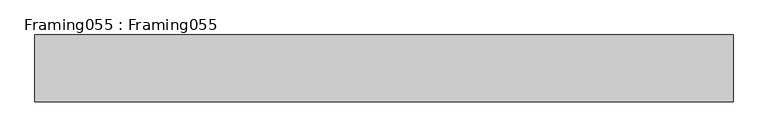
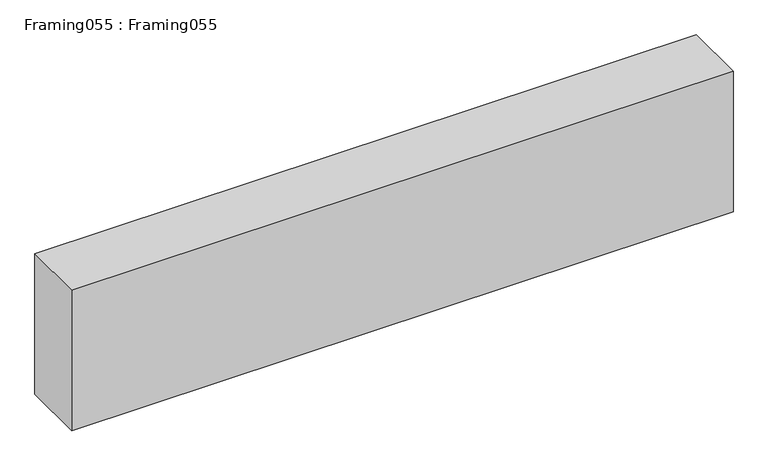
"""IFC4 building model written with IfcOpenShell, lengths in millimetres: proxy geometry, Framing055 : Framing055."""

from ifc_helpers import new_model, si_unit, frame, origin, place, context, project, spatial, polyline, outline, extrude, source, transform, mapped, element, save


def framing055_framing055_ac69ba7b(model_context):
    return source(origin(), model_context, "Body", "SweptSolid", [
        extrude(outline(polyline([(-5503.7121051, 9829.7531721), (-7089.7776325, 9829.7531721), (-7089.7776325, 9982.1531721), (-5503.7121051, 9982.1531721), (-5503.7121051, 9829.7531721)])), frame((0.0, 0.0, 39579.2960083), z_axis=(0.0, 0.0, 1.0), x_axis=(1.0, 0.0, 0.0)), (0.0, 0.0, 1.0), 355.6),
    ])


if __name__ == "__main__":
    model = new_model("IFC4")
    model_context = context("Model", 3, world=origin())
    ifc_project = project(units=[si_unit("LENGTHUNIT", "METRE", prefix="MILLI")], contexts=[model_context])
    site = spatial("IfcSite", under=ifc_project)
    building = spatial("IfcBuilding", under=site)
    placement = place(None, origin())
    framing055_framing055_shape = framing055_framing055_ac69ba7b(model_context)
    element("IfcBuildingElementProxy", 1, Name="Framing055 : Framing055", ObjectType="Framing055 : Framing055", at=placement, inside=building, context=model_context, shape_type="MappedRepresentation", body=[
        mapped(framing055_framing055_shape, transform((0.0, 0.0, 0.0), x_axis=(1.0, 0.0, 0.0), y_axis=(0.0, 1.0, 0.0), z_axis=(0.0, 0.0, 1.0))),
    ])
    save(model, "model.ifc")

# Revit data of these elements
# Type "Framing055 : Framing055"
#   NameOverride = "Framing055"
# Element 1 (IfcBuildingElementProxy, "Framing055 : Framing055")
#   Materials on its faces: "WOOD FRAMING (SEE STRUCT DWGS)"
# Materials
#   "WOOD FRAMING (SEE STRUCT DWGS)": class "Unassigned", colour RGB 224 188 168, transparency 0, Cost = 0
